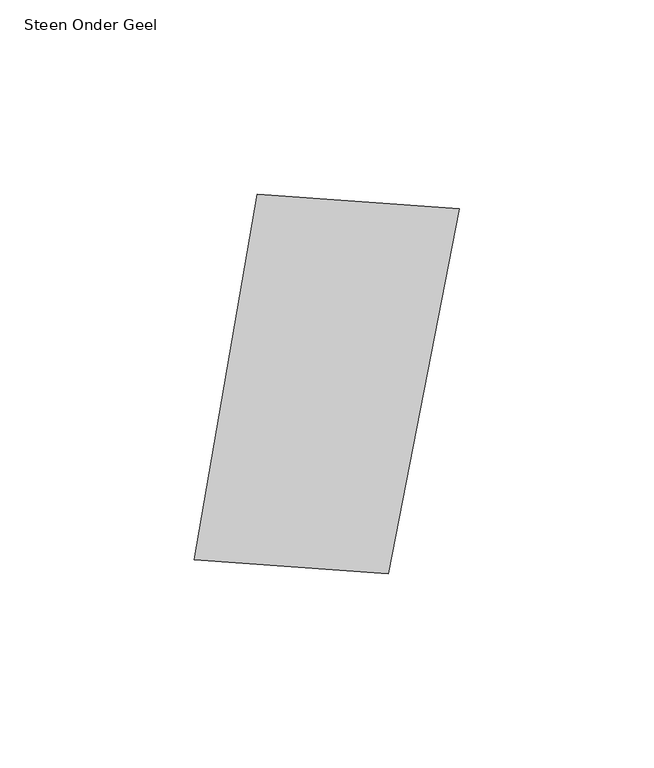
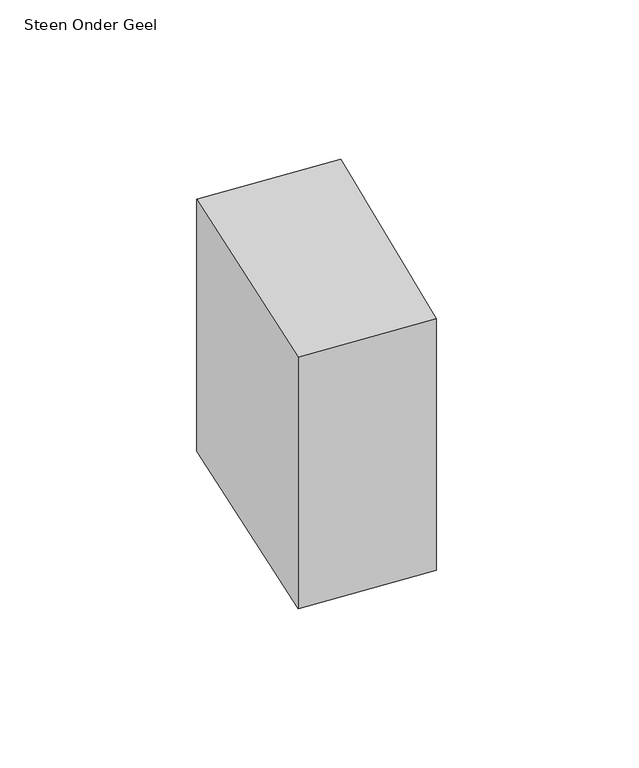
"""IFC4 building model written with IfcOpenShell, lengths in millimetres: proxy geometry, 00_GMA_steen_versie_4 : Steen Onder Geel."""

from ifc_helpers import new_model, si_unit, origin, origin_with_axes, place, context, project, spatial, polyline, outline, extrude, source, transform, mapped, element, save


def steen_onder_geel_77b23767(model_context):
    return source(origin(), model_context, "Body", "SweptSolid", [
        extrude(outline(polyline([(109.26181, 113.4821274), (90.9114369, 19.5139431), (41.0382455, 23.0727052), (57.2801105, 117.1811514), (109.26181, 113.4821274)])), origin_with_axes(), (0.0, 0.0, 1.0), 100.0),
    ])


if __name__ == "__main__":
    model = new_model("IFC4")
    model_context = context("Model", 3, world=origin())
    ifc_project = project(units=[si_unit("LENGTHUNIT", "METRE", prefix="MILLI")], contexts=[model_context])
    site = spatial("IfcSite", under=ifc_project)
    building = spatial("IfcBuilding", under=site)
    placement = place(None, origin())
    steen_onder_geel_shape = steen_onder_geel_77b23767(model_context)
    element("IfcBuildingElementProxy", 1, Name="00_GMA_steen_versie_4 : Steen Onder Geel", ObjectType="00_GMA_steen_versie_4 : Steen Onder Geel", at=placement, inside=building, context=model_context, shape_type="MappedRepresentation", body=[
        mapped(steen_onder_geel_shape, transform((0.0, 0.0, 0.0), x_axis=(1.0, 0.0, 0.0), y_axis=(0.0, 1.0, 0.0), z_axis=(0.0, 0.0, 1.0))),
    ])
    save(model, "model.ifc")

# Revit data of these elements
# Type "00_GMA_steen_versie_4 : Steen Onder Geel"
#   StootVoegHalfBoven [instance default] = 5 mm
#   StootVoegHalf [instance default] = 5 mm
#   StootVoegBreedteOnder = 10 mm
#   StootVoegBreedteBoven = 10 mm
#   Steendikte = 100 mm
#   LintVoegOnderHalf = 0 mm
#   LintVoegOnder = 0 mm
#   LintVoegBovenHalf = 5 mm
#   LintVoegBoven = 10 mm
#   materiaal = 21_steen_geel
#   MateriaalVoeg = none
#   Default Elevation = 0
# Element 1 (IfcBuildingElementProxy, "00_GMA_steen_versie_4 : Steen Onder Geel")
#   Materials on its faces: "21_steen_geel"
# Materials
#   "21_steen_geel": class "Unassigned", colour RGB 202 202 0, transparency 0, Cost = 0
